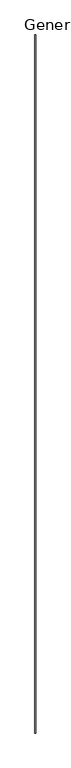
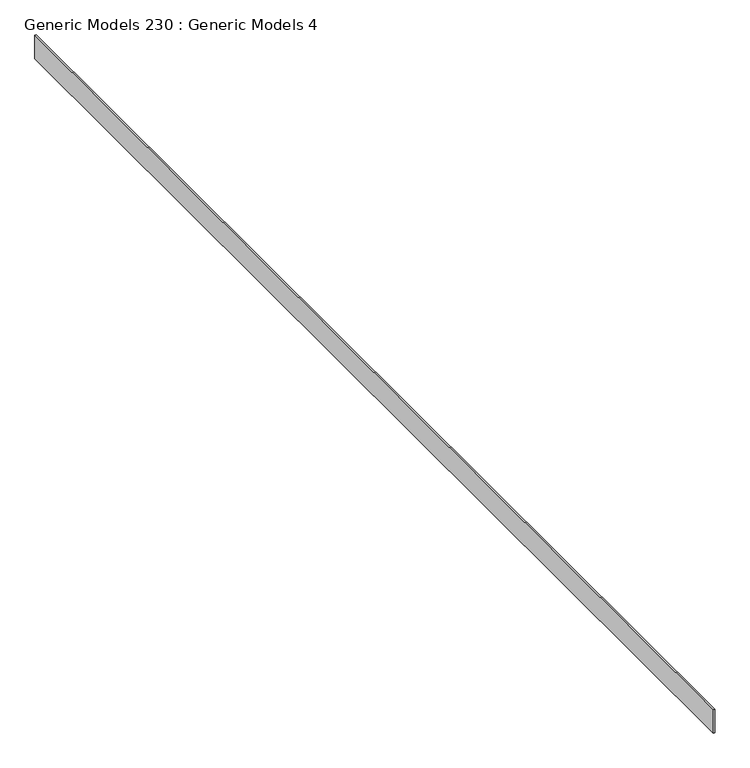
"""IFC4 building model written with IfcOpenShell, lengths in millimetres: proxy geometry, Generic Models 230 : Generic Models 4."""

from ifc_helpers import new_model, si_unit, frame, origin, place, context, project, spatial, polyline, outline, extrude, source, transform, mapped, element, save


def generic_models_230_generic_models_4_e46a4a02(model_context):
    return source(origin(), model_context, "Body", "SweptSolid", [
        extrude(outline(polyline([(7253.8514146, -6864.9230338), (7234.8014146, -6864.9230338), (7234.8014146, 11778.6769662), (7253.8514146, 11778.6769662), (7253.8514146, -6864.9230338)])), frame((0.0, 0.0, 126809.341198), z_axis=(0.0, 0.0, 1.0), x_axis=(1.0, 0.0, 0.0)), (0.0, 0.0, 1.0), 389.1918058),
    ])


if __name__ == "__main__":
    model = new_model("IFC4")
    model_context = context("Model", 3, world=origin())
    ifc_project = project(units=[si_unit("LENGTHUNIT", "METRE", prefix="MILLI")], contexts=[model_context])
    site = spatial("IfcSite", under=ifc_project)
    building = spatial("IfcBuilding", under=site)
    placement = place(None, origin())
    generic_models_230_generic_models_4_shape = generic_models_230_generic_models_4_e46a4a02(model_context)
    element("IfcBuildingElementProxy", 1, Name="Generic Models 230 : Generic Models 4", ObjectType="Generic Models 230 : Generic Models 4", at=placement, inside=building, context=model_context, shape_type="MappedRepresentation", body=[
        mapped(generic_models_230_generic_models_4_shape, transform((0.0, 0.0, 0.0), x_axis=(1.0, 0.0, 0.0), y_axis=(0.0, 1.0, 0.0), z_axis=(0.0, 0.0, 1.0))),
    ])
    save(model, "model.ifc")

# Revit data of these elements
# Element 1 (IfcBuildingElementProxy, "Generic Models 230 : Generic Models 4")
#   Materials on its faces: "_CDX PLYWOOD - SEE STRUCT DWGs"
# Materials
#   "_CDX PLYWOOD - SEE STRUCT DWGs": class "Generic", colour RGB 98 75 74, transparency 0, Cost = 0
